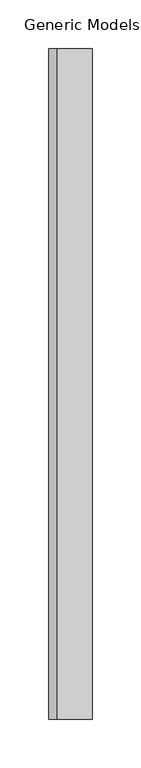
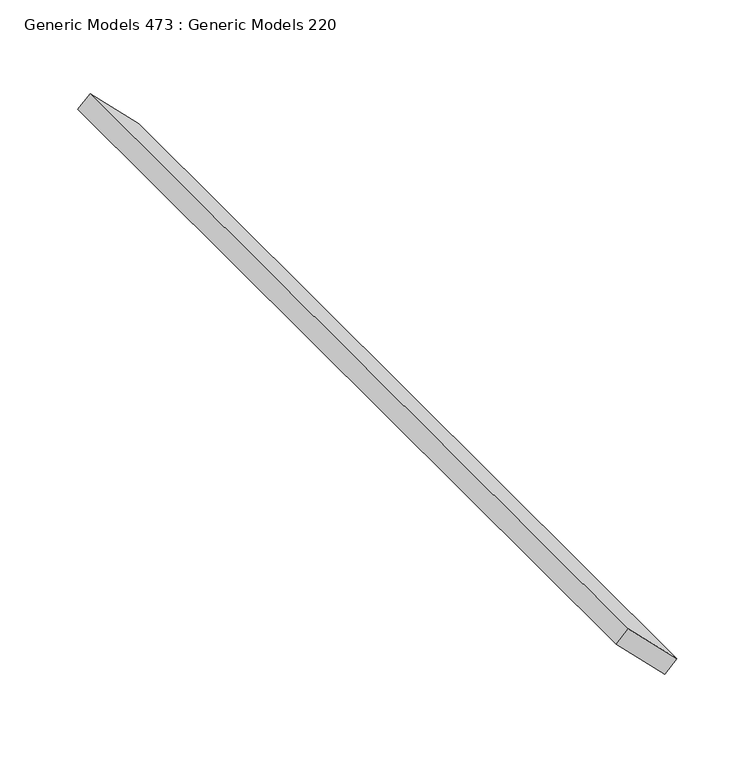
"""IFC4 building model written with IfcOpenShell, lengths in millimetres: proxy geometry, Generic Models 473 : Generic Models 220."""

from ifc_helpers import new_model, si_unit, frame, origin, place, context, project, spatial, polyline, outline, extrude, source, transform, mapped, element, save


def generic_models_473_generic_models_220_40795c9d(model_context):
    return source(origin(), model_context, "Body", "SweptSolid", [
        extrude(outline(polyline([(0.0, -50.8), (0.0, 0.0), (690.8142348, 0.0), (690.8142348, -50.8), (0.0, -50.8)])), frame((-6899.085451, -4564.8872686, 128069.1762561), z_axis=(0.7071067811865582, 0.0, 0.7071067811865369), x_axis=(0.0, 1.0, 0.0)), (0.0, 0.0, 1.0), 12.7),
    ])


if __name__ == "__main__":
    model = new_model("IFC4")
    model_context = context("Model", 3, world=origin())
    ifc_project = project(units=[si_unit("LENGTHUNIT", "METRE", prefix="MILLI")], contexts=[model_context])
    site = spatial("IfcSite", under=ifc_project)
    building = spatial("IfcBuilding", under=site)
    placement = place(None, origin())
    generic_models_473_generic_models_220_shape = generic_models_473_generic_models_220_40795c9d(model_context)
    element("IfcBuildingElementProxy", 1, Name="Generic Models 473 : Generic Models 220", ObjectType="Generic Models 473 : Generic Models 220", at=placement, inside=building, context=model_context, shape_type="MappedRepresentation", body=[
        mapped(generic_models_473_generic_models_220_shape, transform((0.0, 0.0, 0.0), x_axis=(1.0, 0.0, 0.0), y_axis=(0.0, 1.0, 0.0), z_axis=(0.0, 0.0, 1.0))),
    ])
    save(model, "model.ifc")

# Revit data of these elements
# Element 1 (IfcBuildingElementProxy, "Generic Models 473 : Generic Models 220")
#   Materials on its faces: "_WOOD TONE ALUMINUM EXTRUSION SLAT BY KNOTWOOD"
# Materials
#   "_WOOD TONE ALUMINUM EXTRUSION SLAT BY KNOTWOOD": class "Generic", colour RGB 177 130 114, transparency 0, Cost = 0
